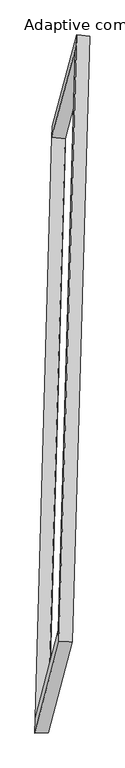
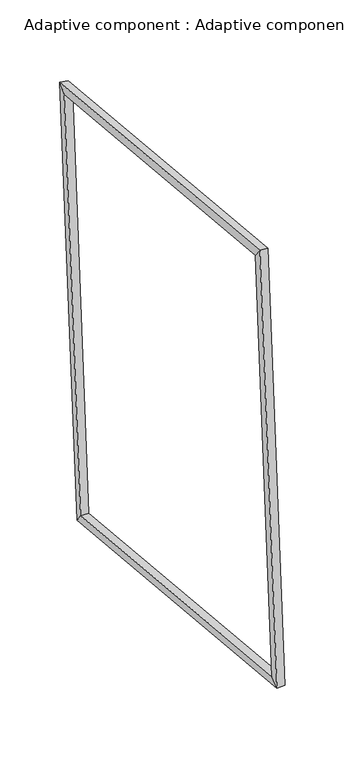
"""IFC4 building model written with IfcOpenShell, lengths in millimetres: proxy geometry, Adaptive component : Adaptive component."""

import ifcopenshell
import ifcopenshell.guid

model = None  # the IFC model being written
_history = None  # IfcOwnerHistory: only IFC2X3 demands one
_inside = {}  # id of a spatial element -> (the spatial element, [elements in it])
_under = {}  # id of a project, library or spatial element -> (it, [spatial elements below it])
_declared = {}  # id of a project -> (the project, [libraries it declares])
_typed = {}  # id of a type object -> (the type object, [elements of that type])
_made_of = {}  # id of a material, layer set ... -> (it, [elements and type objects made of it])


def new_model(schema):
    """Start an empty IFC model of exactly this schema.

    Asked for "IFC4X3", IfcOpenShell would pick the latest addendum, in which some entities
    have other attributes; the version numbers below select the first issue.
    IFC2X3 requires an IfcOwnerHistory on every rooted entity: one is made here for all.
    """
    global model, _history
    if schema == "IFC4X3":
        model = ifcopenshell.file(schema_version=(4, 3, 0, 0))
    else:
        model = ifcopenshell.file(schema=schema)
    _inside.clear()
    _under.clear()
    _declared.clear()
    _typed.clear()
    _made_of.clear()
    _history = None
    if model.schema == "IFC2X3":
        org = make("IfcOrganization", Name="unknown")
        user = make(
            "IfcPersonAndOrganization",
            ThePerson=make("IfcPerson", FamilyName="unknown"),
            TheOrganization=org,
        )
        app = make(
            "IfcApplication",
            ApplicationDeveloper=org,
            Version="unknown",
            ApplicationFullName="unknown",
            ApplicationIdentifier="unknown",
        )
        _history = make(
            "IfcOwnerHistory",
            OwningUser=user,
            OwningApplication=app,
            ChangeAction="ADDED",
            CreationDate=0,
        )
    return model


def make(cls, **values):
    """One entity of the class cls with the attributes given. An attribute that is None is left unset."""
    return model.create_entity(
        cls, **{name: value for name, value in values.items() if value is not None}
    )


def rooted(cls, **values):
    """An entity with a GlobalId (a new one), such as an element, a storey or a relation."""
    return make(cls, GlobalId=ifcopenshell.guid.new(), OwnerHistory=_history, **values)


def si_unit(unit_type, name, prefix=None):
    """IfcSIUnit, for example si_unit("LENGTHUNIT", "METRE", prefix="MILLI")."""
    return make("IfcSIUnit", UnitType=unit_type, Prefix=prefix, Name=name)


def assignment(units):
    """IfcUnitAssignment: the units of a project."""
    return None if units is None else make("IfcUnitAssignment", Units=units)


def point(xyz):
    """IfcCartesianPoint."""
    return None if xyz is None else make("IfcCartesianPoint", Coordinates=xyz)


def direction(xyz):
    """IfcDirection."""
    return None if xyz is None else make("IfcDirection", DirectionRatios=xyz)


def frame(location, z_axis=None, x_axis=None):
    """IfcAxis2Placement3D, a coordinate frame: its origin and axes. An axis left out is left unset."""
    return make(
        "IfcAxis2Placement3D",
        Location=point(location),
        Axis=direction(z_axis),
        RefDirection=direction(x_axis),
    )


def origin():
    """The frame at (0, 0, 0) with its axes left unset."""
    return frame((0.0, 0.0, 0.0))


def place(relative_to, where):
    """IfcLocalPlacement: puts the frame where relative to a parent placement (None: the world)."""
    return make(
        "IfcLocalPlacement", PlacementRelTo=relative_to, RelativePlacement=where
    )


def context(
    kind, dimensions, precision=None, world=None, true_north=None, identifier=None
):
    """IfcGeometricRepresentationContext, for example the 3D "Model" context."""
    return make(
        "IfcGeometricRepresentationContext",
        ContextIdentifier=identifier,
        ContextType=kind,
        CoordinateSpaceDimension=dimensions,
        Precision=precision,
        WorldCoordinateSystem=world,
        TrueNorth=true_north,
    )


def project(units=None, contexts=None):
    """IfcProject with its units and contexts."""
    return rooted(
        "IfcProject",
        Name="project",
        RepresentationContexts=contexts,
        UnitsInContext=assignment(units),
    )


def spatial(cls, under=None, at=None, **own):
    """A site, building, storey or space (cls), placed at a placement, below another one or the project."""
    s = rooted(cls, ObjectPlacement=at, **own)
    if under is not None:
        _under.setdefault(under.id(), (under, []))[1].append(s)
    return s


def faces_of(points, faces, orient=None, outer=None):
    """IfcFace entities. A face is a list of loops; a loop is a list of indices into points, from 0.

    orient and outer hold one flag for each loop. By default every Orientation is true, the
    first loop of a face is its IfcFaceOuterBound and the others are IfcFaceBound.
    """
    made = []
    for i, loops in enumerate(faces):
        bounds = []
        for j, loop in enumerate(loops):
            is_outer = j == 0 if outer is None else outer[i][j]
            bounds.append(
                make(
                    "IfcFaceOuterBound" if is_outer else "IfcFaceBound",
                    Bound=make("IfcPolyLoop", Polygon=[points[k] for k in loop]),
                    Orientation=True if orient is None else orient[i][j],
                )
            )
        made.append(make("IfcFace", Bounds=bounds))
    return made


def faceted_brep(points, faces, orient=None, outer=None, voids=None):
    """IfcFacetedBrep: a solid bounded by flat faces; with voids (closed shells), ...WithVoids."""
    shared = [point(p) for p in points]
    hull = make("IfcClosedShell", CfsFaces=faces_of(shared, faces, orient, outer))
    if voids is None:
        return make("IfcFacetedBrep", Outer=hull)
    return make(
        "IfcFacetedBrepWithVoids",
        Outer=hull,
        Voids=[
            make(cls, CfsFaces=faces_of(shared, fs, o, b)) for cls, fs, o, b in voids
        ],
    )


def shape(context_of_items, identifier, shape_type, items):
    """IfcShapeRepresentation: the items that make up one representation, for example the "Body"."""
    return make(
        "IfcShapeRepresentation",
        ContextOfItems=context_of_items,
        RepresentationIdentifier=identifier,
        RepresentationType=shape_type,
        Items=items,
    )


def source(mapping_origin, context_of_items, identifier, shape_type, items):
    """IfcRepresentationMap: a shape defined once, which mapped items show again and again."""
    return make(
        "IfcRepresentationMap",
        MappingOrigin=mapping_origin,
        MappedRepresentation=shape(context_of_items, identifier, shape_type, items),
    )


def transform(
    local_origin,
    x_axis=None,
    y_axis=None,
    z_axis=None,
    scale=None,
    scale2=None,
    scale3=None,
    uniform=True,
):
    """IfcCartesianTransformationOperator3D, or its non-uniform kind. x_axis, y_axis, z_axis: its Axis1, 2, 3."""
    if uniform:
        return make(
            "IfcCartesianTransformationOperator3D",
            Axis1=direction(x_axis),
            Axis2=direction(y_axis),
            LocalOrigin=point(local_origin),
            Scale=scale,
            Axis3=direction(z_axis),
        )
    return make(
        "IfcCartesianTransformationOperator3DnonUniform",
        Axis1=direction(x_axis),
        Axis2=direction(y_axis),
        LocalOrigin=point(local_origin),
        Scale=scale,
        Axis3=direction(z_axis),
        Scale2=scale2,
        Scale3=scale3,
    )


def mapped(mapping_source, mapping_target):
    """IfcMappedItem: shows the shape of a source again, moved by a transform."""
    return make(
        "IfcMappedItem", MappingSource=mapping_source, MappingTarget=mapping_target
    )


def made_of(thing, what):
    """Note that an element or type object is made of a material, layer set ...; save() writes the relation."""
    if what is not None:
        _made_of.setdefault(what.id(), (what, []))[1].append(thing)
    return thing


def element(
    cls,
    number,
    at=None,
    inside=None,
    cuts=None,
    type_object=None,
    material=None,
    context=None,
    identifier="Body",
    shape_type=None,
    held_by="IfcProductDefinitionShape",
    body=None,
    shapes=None,
    **own,
):
    """One element of the class cls, such as IfcWall. Its Tag is "e" and its number.

    at: its placement. inside: the storey or other place that contains it. cuts: it is an
    opening in that element (IfcRelVoidsElement). A single representation is given by context,
    identifier, shape_type and body (its items); several are given by shapes. held_by: the class
    of the entity that holds the representations. save() writes the other relations.
    """
    e = rooted(cls, Tag="e%d" % number, ObjectPlacement=at, **own)
    if body is not None:
        shapes = [shape(context, identifier, shape_type, body)]
    if shapes is not None:
        e.Representation = make(held_by, Representations=shapes)
    if inside is not None:
        _inside.setdefault(inside.id(), (inside, []))[1].append(e)
    if cuts is not None:
        rooted(
            "IfcRelVoidsElement", RelatingBuildingElement=cuts, RelatedOpeningElement=e
        )
    if type_object is not None:
        _typed.setdefault(type_object.id(), (type_object, []))[1].append(e)
    return made_of(e, material)


def aggregate(whole, parts):
    """IfcRelAggregates: a whole, such as a stair, and the parts it consists of."""
    return rooted("IfcRelAggregates", RelatingObject=whole, RelatedObjects=parts)


def save(model, path):
    """Write the relations noted so far, then the file.

    IfcRelAggregates (storeys below a building ...), IfcRelContainedInSpatialStructure (elements
    in a storey), IfcRelDefinesByType, IfcRelAssociatesMaterial and IfcRelDeclares: one each for
    every whole, place, type object, material and project.
    """
    for whole, parts in _under.values():
        aggregate(whole, parts)
    for where, things in _inside.values():
        rooted(
            "IfcRelContainedInSpatialStructure",
            RelatedElements=things,
            RelatingStructure=where,
        )
    for kind, things in _typed.values():
        rooted("IfcRelDefinesByType", RelatedObjects=things, RelatingType=kind)
    for what, things in _made_of.values():
        rooted("IfcRelAssociatesMaterial", RelatedObjects=things, RelatingMaterial=what)
    for by, libraries in _declared.values():
        rooted("IfcRelDeclares", RelatingContext=by, RelatedDefinitions=libraries)
    model.write(path)


def adaptive_component_adaptive_component_c6baadc9(model_context):
    return source(origin(), model_context, "Body", "Brep", [
        faceted_brep([(74.9939983, 1225.9349657, 2832.3498292), (139.6345509, 1220.0591686, 2827.5254813), (57.0410273, -1631.8931089, 3198.4818024), (-7.7916696, -1632.6520507, 3204.1691375), (82.3971029, 1298.4756745, 2888.2232509), (-4.1154723, -1688.8013568, 3276.7813998), (147.0376554, 1292.5998774, 2883.398903), (60.7172245, -1688.042415, 3271.0940647), (-56.869824, -2062.667446, -138.7201267), (-121.9289808, -2064.2827868, -139.6673016), (-122.6452908, -2137.0431476, -195.7406147), (-57.5861339, -2135.4278067, -194.7934398), (25.7236996, 789.2848315, -509.6764478), (-39.1433129, 794.3042295, -511.4866099), (-36.1327155, 850.2338837, -584.2987636), (28.734297, 845.2144857, -582.4886015)], [[[0, 1, 2, 3]], [[4, 0, 3, 5]], [[6, 4, 5, 7]], [[1, 6, 7, 2]], [[3, 2, 8, 9]], [[5, 3, 9, 10]], [[7, 5, 10, 11]], [[2, 7, 11, 8]], [[9, 8, 12, 13]], [[10, 9, 13, 14]], [[11, 10, 14, 15]], [[8, 11, 15, 12]], [[13, 12, 1, 0]], [[14, 13, 0, 4]], [[15, 14, 4, 6]], [[12, 15, 6, 1]]]),
    ])


if __name__ == "__main__":
    model = new_model("IFC4")
    model_context = context("Model", 3, world=origin())
    ifc_project = project(units=[si_unit("LENGTHUNIT", "METRE", prefix="MILLI")], contexts=[model_context])
    site = spatial("IfcSite", under=ifc_project)
    building = spatial("IfcBuilding", under=site)
    placement = place(None, origin())
    adaptive_component_adaptive_component_shape = adaptive_component_adaptive_component_c6baadc9(model_context)
    element("IfcBuildingElementProxy", 1, Name="Adaptive component : Adaptive component", ObjectType="Adaptive component : Adaptive component", at=placement, inside=building, context=model_context, shape_type="MappedRepresentation", body=[
        mapped(adaptive_component_adaptive_component_shape, transform((0.0, 0.0, 0.0), x_axis=(1.0, 0.0, 0.0), y_axis=(0.0, 1.0, 0.0), z_axis=(0.0, 0.0, 1.0))),
    ])
    save(model, "model.ifc")

# Revit data of these elements
# Type "Adaptive component : Adaptive component"
#   r [instance default] = 2063.125 mm
#   2r [instance default] = 4126.251 mm
#   Number [instance default] = 5
#   Default Elevation = 0
# Element 1 (IfcBuildingElementProxy, "Adaptive component : Adaptive component")
#   r = 2308.256 mm
#   2r = 4616.511 mm
#   Number = 14
